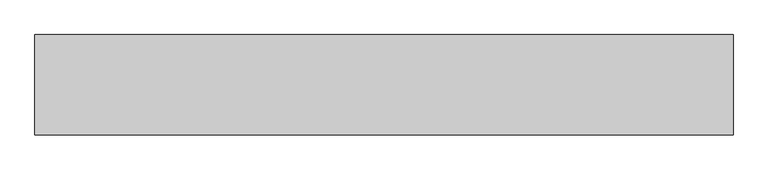
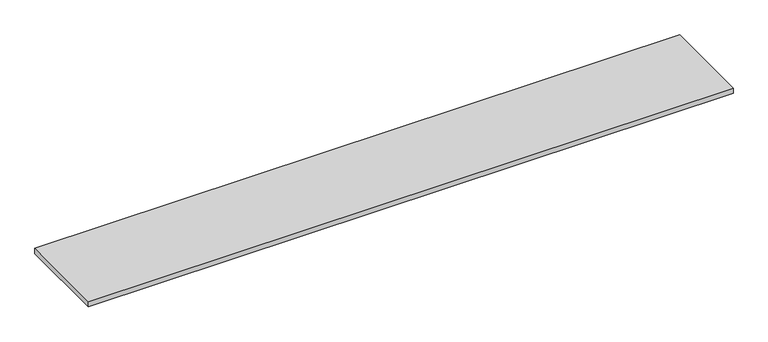
"""IFC4 building model written with IfcOpenShell, lengths in millimetres: furniture geometry, OD_CW_Countertop : OD_CW_Countertop."""

import ifcopenshell
import ifcopenshell.guid

model = None  # the IFC model being written
_history = None  # IfcOwnerHistory: only IFC2X3 demands one
_inside = {}  # id of a spatial element -> (the spatial element, [elements in it])
_under = {}  # id of a project, library or spatial element -> (it, [spatial elements below it])
_declared = {}  # id of a project -> (the project, [libraries it declares])
_typed = {}  # id of a type object -> (the type object, [elements of that type])
_made_of = {}  # id of a material, layer set ... -> (it, [elements and type objects made of it])


def new_model(schema):
    """Start an empty IFC model of exactly this schema.

    Asked for "IFC4X3", IfcOpenShell would pick the latest addendum, in which some entities
    have other attributes; the version numbers below select the first issue.
    IFC2X3 requires an IfcOwnerHistory on every rooted entity: one is made here for all.
    """
    global model, _history
    if schema == "IFC4X3":
        model = ifcopenshell.file(schema_version=(4, 3, 0, 0))
    else:
        model = ifcopenshell.file(schema=schema)
    _inside.clear()
    _under.clear()
    _declared.clear()
    _typed.clear()
    _made_of.clear()
    _history = None
    if model.schema == "IFC2X3":
        org = make("IfcOrganization", Name="unknown")
        user = make(
            "IfcPersonAndOrganization",
            ThePerson=make("IfcPerson", FamilyName="unknown"),
            TheOrganization=org,
        )
        app = make(
            "IfcApplication",
            ApplicationDeveloper=org,
            Version="unknown",
            ApplicationFullName="unknown",
            ApplicationIdentifier="unknown",
        )
        _history = make(
            "IfcOwnerHistory",
            OwningUser=user,
            OwningApplication=app,
            ChangeAction="ADDED",
            CreationDate=0,
        )
    return model


def make(cls, **values):
    """One entity of the class cls with the attributes given. An attribute that is None is left unset."""
    return model.create_entity(
        cls, **{name: value for name, value in values.items() if value is not None}
    )


def rooted(cls, **values):
    """An entity with a GlobalId (a new one), such as an element, a storey or a relation."""
    return make(cls, GlobalId=ifcopenshell.guid.new(), OwnerHistory=_history, **values)


def si_unit(unit_type, name, prefix=None):
    """IfcSIUnit, for example si_unit("LENGTHUNIT", "METRE", prefix="MILLI")."""
    return make("IfcSIUnit", UnitType=unit_type, Prefix=prefix, Name=name)


def assignment(units):
    """IfcUnitAssignment: the units of a project."""
    return None if units is None else make("IfcUnitAssignment", Units=units)


def point(xyz):
    """IfcCartesianPoint."""
    return None if xyz is None else make("IfcCartesianPoint", Coordinates=xyz)


def direction(xyz):
    """IfcDirection."""
    return None if xyz is None else make("IfcDirection", DirectionRatios=xyz)


def frame(location, z_axis=None, x_axis=None):
    """IfcAxis2Placement3D, a coordinate frame: its origin and axes. An axis left out is left unset."""
    return make(
        "IfcAxis2Placement3D",
        Location=point(location),
        Axis=direction(z_axis),
        RefDirection=direction(x_axis),
    )


def origin():
    """The frame at (0, 0, 0) with its axes left unset."""
    return frame((0.0, 0.0, 0.0))


def place(relative_to, where):
    """IfcLocalPlacement: puts the frame where relative to a parent placement (None: the world)."""
    return make(
        "IfcLocalPlacement", PlacementRelTo=relative_to, RelativePlacement=where
    )


def context(
    kind, dimensions, precision=None, world=None, true_north=None, identifier=None
):
    """IfcGeometricRepresentationContext, for example the 3D "Model" context."""
    return make(
        "IfcGeometricRepresentationContext",
        ContextIdentifier=identifier,
        ContextType=kind,
        CoordinateSpaceDimension=dimensions,
        Precision=precision,
        WorldCoordinateSystem=world,
        TrueNorth=true_north,
    )


def project(units=None, contexts=None):
    """IfcProject with its units and contexts."""
    return rooted(
        "IfcProject",
        Name="project",
        RepresentationContexts=contexts,
        UnitsInContext=assignment(units),
    )


def spatial(cls, under=None, at=None, **own):
    """A site, building, storey or space (cls), placed at a placement, below another one or the project."""
    s = rooted(cls, ObjectPlacement=at, **own)
    if under is not None:
        _under.setdefault(under.id(), (under, []))[1].append(s)
    return s


def polyline(points):
    """IfcPolyline through the points."""
    return make("IfcPolyline", Points=[point(p) for p in points])


def outline(outer, holes=None, kind="AREA"):
    """IfcArbitraryClosedProfileDef: a profile drawn as a closed curve; with holes, ...WithVoids."""
    if holes is None:
        return make("IfcArbitraryClosedProfileDef", ProfileType=kind, OuterCurve=outer)
    return make(
        "IfcArbitraryProfileDefWithVoids",
        ProfileType=kind,
        OuterCurve=outer,
        InnerCurves=holes,
    )


def extrude(swept, where, along, depth):
    """IfcExtrudedAreaSolid: the profile swept, set in the frame where, extruded along a direction by depth."""
    return make(
        "IfcExtrudedAreaSolid",
        SweptArea=swept,
        Position=where,
        ExtrudedDirection=direction(along),
        Depth=depth,
    )


def shape(context_of_items, identifier, shape_type, items):
    """IfcShapeRepresentation: the items that make up one representation, for example the "Body"."""
    return make(
        "IfcShapeRepresentation",
        ContextOfItems=context_of_items,
        RepresentationIdentifier=identifier,
        RepresentationType=shape_type,
        Items=items,
    )


def source(mapping_origin, context_of_items, identifier, shape_type, items):
    """IfcRepresentationMap: a shape defined once, which mapped items show again and again."""
    return make(
        "IfcRepresentationMap",
        MappingOrigin=mapping_origin,
        MappedRepresentation=shape(context_of_items, identifier, shape_type, items),
    )


def transform(
    local_origin,
    x_axis=None,
    y_axis=None,
    z_axis=None,
    scale=None,
    scale2=None,
    scale3=None,
    uniform=True,
):
    """IfcCartesianTransformationOperator3D, or its non-uniform kind. x_axis, y_axis, z_axis: its Axis1, 2, 3."""
    if uniform:
        return make(
            "IfcCartesianTransformationOperator3D",
            Axis1=direction(x_axis),
            Axis2=direction(y_axis),
            LocalOrigin=point(local_origin),
            Scale=scale,
            Axis3=direction(z_axis),
        )
    return make(
        "IfcCartesianTransformationOperator3DnonUniform",
        Axis1=direction(x_axis),
        Axis2=direction(y_axis),
        LocalOrigin=point(local_origin),
        Scale=scale,
        Axis3=direction(z_axis),
        Scale2=scale2,
        Scale3=scale3,
    )


def mapped(mapping_source, mapping_target):
    """IfcMappedItem: shows the shape of a source again, moved by a transform."""
    return make(
        "IfcMappedItem", MappingSource=mapping_source, MappingTarget=mapping_target
    )


def made_of(thing, what):
    """Note that an element or type object is made of a material, layer set ...; save() writes the relation."""
    if what is not None:
        _made_of.setdefault(what.id(), (what, []))[1].append(thing)
    return thing


def element(
    cls,
    number,
    at=None,
    inside=None,
    cuts=None,
    type_object=None,
    material=None,
    context=None,
    identifier="Body",
    shape_type=None,
    held_by="IfcProductDefinitionShape",
    body=None,
    shapes=None,
    **own,
):
    """One element of the class cls, such as IfcWall. Its Tag is "e" and its number.

    at: its placement. inside: the storey or other place that contains it. cuts: it is an
    opening in that element (IfcRelVoidsElement). A single representation is given by context,
    identifier, shape_type and body (its items); several are given by shapes. held_by: the class
    of the entity that holds the representations. save() writes the other relations.
    """
    e = rooted(cls, Tag="e%d" % number, ObjectPlacement=at, **own)
    if body is not None:
        shapes = [shape(context, identifier, shape_type, body)]
    if shapes is not None:
        e.Representation = make(held_by, Representations=shapes)
    if inside is not None:
        _inside.setdefault(inside.id(), (inside, []))[1].append(e)
    if cuts is not None:
        rooted(
            "IfcRelVoidsElement", RelatingBuildingElement=cuts, RelatedOpeningElement=e
        )
    if type_object is not None:
        _typed.setdefault(type_object.id(), (type_object, []))[1].append(e)
    return made_of(e, material)


def aggregate(whole, parts):
    """IfcRelAggregates: a whole, such as a stair, and the parts it consists of."""
    return rooted("IfcRelAggregates", RelatingObject=whole, RelatedObjects=parts)


def save(model, path):
    """Write the relations noted so far, then the file.

    IfcRelAggregates (storeys below a building ...), IfcRelContainedInSpatialStructure (elements
    in a storey), IfcRelDefinesByType, IfcRelAssociatesMaterial and IfcRelDeclares: one each for
    every whole, place, type object, material and project.
    """
    for whole, parts in _under.values():
        aggregate(whole, parts)
    for where, things in _inside.values():
        rooted(
            "IfcRelContainedInSpatialStructure",
            RelatedElements=things,
            RelatingStructure=where,
        )
    for kind, things in _typed.values():
        rooted("IfcRelDefinesByType", RelatedObjects=things, RelatingType=kind)
    for what, things in _made_of.values():
        rooted("IfcRelAssociatesMaterial", RelatedObjects=things, RelatingMaterial=what)
    for by, libraries in _declared.values():
        rooted("IfcRelDeclares", RelatingContext=by, RelatedDefinitions=libraries)
    model.write(path)


def furniture_1b7fe929(model_context):
    return source(origin(), model_context, "Body", "SweptSolid", [
        extrude(outline(polyline([(18.7377049, -609.6), (18.7377049, 25.4), (4438.3377049, 25.4), (4438.3377049, -609.6), (18.7377049, -609.6)])), frame((0.0, 0.0, 965.2), z_axis=(0.0, 0.0, 1.0), x_axis=(1.0, 0.0, 0.0)), (0.0, 0.0, 1.0), 38.1),
    ])


if __name__ == "__main__":
    model = new_model("IFC4")
    model_context = context("Model", 3, world=origin())
    ifc_project = project(units=[si_unit("LENGTHUNIT", "METRE", prefix="MILLI")], contexts=[model_context])
    site = spatial("IfcSite", under=ifc_project)
    building = spatial("IfcBuilding", under=site)
    placement = place(None, origin())
    furniture_shape = furniture_1b7fe929(model_context)
    element("IfcFurniture", 1, ObjectType="OD_CW_Countertop : OD_CW_Countertop", at=placement, inside=building, context=model_context, shape_type="MappedRepresentation", body=[
        mapped(furniture_shape, transform((0.0, 0.0, 0.0), x_axis=(1.0, 0.0, 0.0), y_axis=(0.0, 1.0, 0.0), z_axis=(0.0, 0.0, 1.0))),
    ])
    save(model, "model.ifc")

# Revit data of these elements
# Type "OD_CW_Countertop : OD_CW_Countertop"
#   OD_CW_Width [instance default] = 2' - 9"
#   OD_CW_Off Floor [instance default] = 3' - 2"
#   OD_CW_Length [instance default] = 6' - 9"
#   OD_CW_Height [instance default] = 7' - 0"
#   Depth = 2' - 0"
#   Height = 3' - 0"
#   Width = 4' - 0"
#   OD_CW_Material_Countertop [instance default] = none
# Element 1 (IfcFurniture, "OD_CW_Countertop : OD_CW_Countertop")
#   OD_CW_Width = 2' - 1"
#   OD_CW_Length = 14' - 6"
#   OD_CW_Height = 0' - 1 1/2"
#   Materials on its faces: "CASEWORK"
# Materials
#   "CASEWORK": class "Generic", colour RGB 181 181 181, transparency 0, Cost = 0
